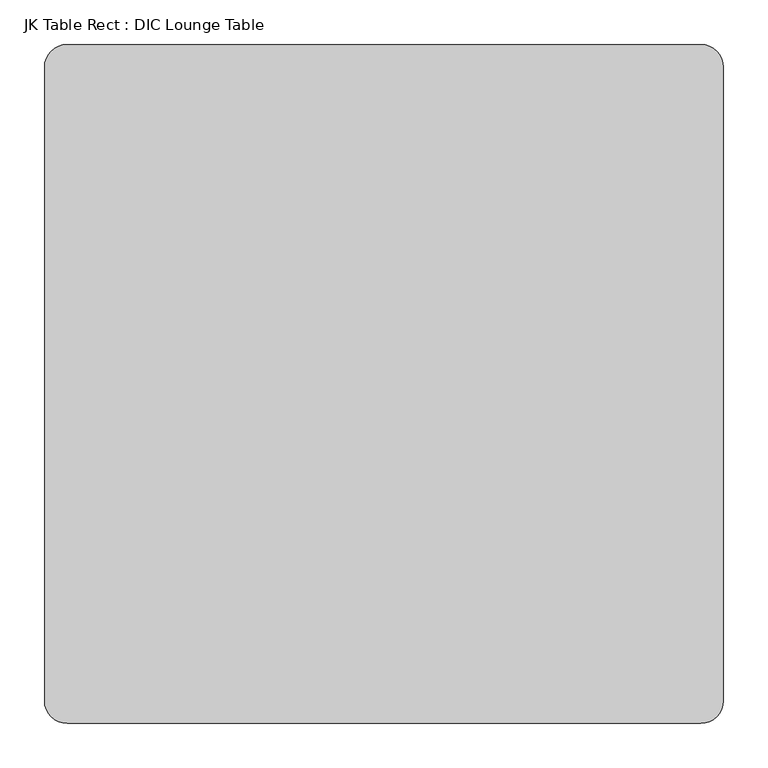
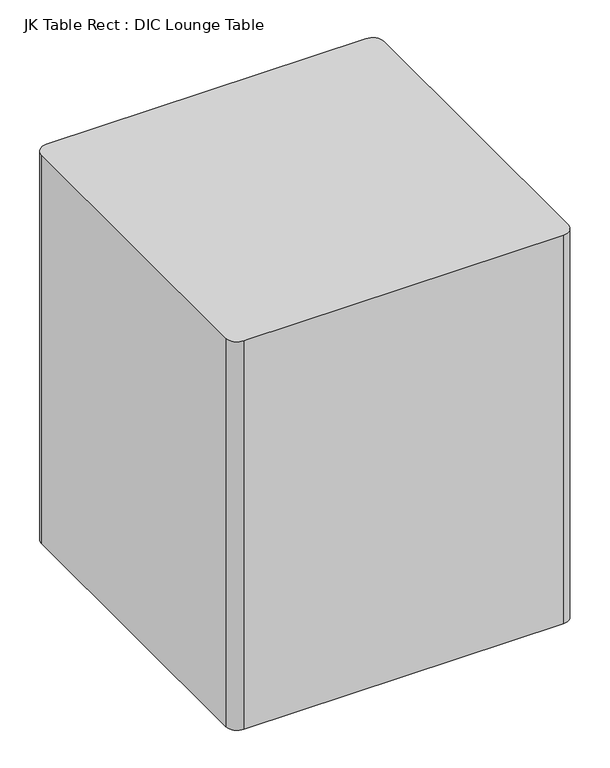
"""IFC4 building model written with IfcOpenShell, lengths in millimetres: furniture geometry, JK Table Rect : DIC Lounge Table."""

import ifcopenshell
import ifcopenshell.guid

model = None  # the IFC model being written
_history = None  # IfcOwnerHistory: only IFC2X3 demands one
_inside = {}  # id of a spatial element -> (the spatial element, [elements in it])
_under = {}  # id of a project, library or spatial element -> (it, [spatial elements below it])
_declared = {}  # id of a project -> (the project, [libraries it declares])
_typed = {}  # id of a type object -> (the type object, [elements of that type])
_made_of = {}  # id of a material, layer set ... -> (it, [elements and type objects made of it])


def new_model(schema):
    """Start an empty IFC model of exactly this schema.

    Asked for "IFC4X3", IfcOpenShell would pick the latest addendum, in which some entities
    have other attributes; the version numbers below select the first issue.
    IFC2X3 requires an IfcOwnerHistory on every rooted entity: one is made here for all.
    """
    global model, _history
    if schema == "IFC4X3":
        model = ifcopenshell.file(schema_version=(4, 3, 0, 0))
    else:
        model = ifcopenshell.file(schema=schema)
    _inside.clear()
    _under.clear()
    _declared.clear()
    _typed.clear()
    _made_of.clear()
    _history = None
    if model.schema == "IFC2X3":
        org = make("IfcOrganization", Name="unknown")
        user = make(
            "IfcPersonAndOrganization",
            ThePerson=make("IfcPerson", FamilyName="unknown"),
            TheOrganization=org,
        )
        app = make(
            "IfcApplication",
            ApplicationDeveloper=org,
            Version="unknown",
            ApplicationFullName="unknown",
            ApplicationIdentifier="unknown",
        )
        _history = make(
            "IfcOwnerHistory",
            OwningUser=user,
            OwningApplication=app,
            ChangeAction="ADDED",
            CreationDate=0,
        )
    return model


def make(cls, **values):
    """One entity of the class cls with the attributes given. An attribute that is None is left unset."""
    return model.create_entity(
        cls, **{name: value for name, value in values.items() if value is not None}
    )


def rooted(cls, **values):
    """An entity with a GlobalId (a new one), such as an element, a storey or a relation."""
    return make(cls, GlobalId=ifcopenshell.guid.new(), OwnerHistory=_history, **values)


def si_unit(unit_type, name, prefix=None):
    """IfcSIUnit, for example si_unit("LENGTHUNIT", "METRE", prefix="MILLI")."""
    return make("IfcSIUnit", UnitType=unit_type, Prefix=prefix, Name=name)


def assignment(units):
    """IfcUnitAssignment: the units of a project."""
    return None if units is None else make("IfcUnitAssignment", Units=units)


def point(xyz):
    """IfcCartesianPoint."""
    return None if xyz is None else make("IfcCartesianPoint", Coordinates=xyz)


def direction(xyz):
    """IfcDirection."""
    return None if xyz is None else make("IfcDirection", DirectionRatios=xyz)


def frame(location, z_axis=None, x_axis=None):
    """IfcAxis2Placement3D, a coordinate frame: its origin and axes. An axis left out is left unset."""
    return make(
        "IfcAxis2Placement3D",
        Location=point(location),
        Axis=direction(z_axis),
        RefDirection=direction(x_axis),
    )


def frame_2d(location, x_axis=None):
    """IfcAxis2Placement2D, a coordinate frame in the plane: its origin and x axis."""
    return make(
        "IfcAxis2Placement2D", Location=point(location), RefDirection=direction(x_axis)
    )


def origin():
    """The frame at (0, 0, 0) with its axes left unset."""
    return frame((0.0, 0.0, 0.0))


def origin_with_axes():
    """The frame at (0, 0, 0) with the z axis (0, 0, 1) and the x axis (1, 0, 0) written out."""
    return frame((0.0, 0.0, 0.0), z_axis=(0.0, 0.0, 1.0), x_axis=(1.0, 0.0, 0.0))


def place(relative_to, where):
    """IfcLocalPlacement: puts the frame where relative to a parent placement (None: the world)."""
    return make(
        "IfcLocalPlacement", PlacementRelTo=relative_to, RelativePlacement=where
    )


def context(
    kind, dimensions, precision=None, world=None, true_north=None, identifier=None
):
    """IfcGeometricRepresentationContext, for example the 3D "Model" context."""
    return make(
        "IfcGeometricRepresentationContext",
        ContextIdentifier=identifier,
        ContextType=kind,
        CoordinateSpaceDimension=dimensions,
        Precision=precision,
        WorldCoordinateSystem=world,
        TrueNorth=true_north,
    )


def project(units=None, contexts=None):
    """IfcProject with its units and contexts."""
    return rooted(
        "IfcProject",
        Name="project",
        RepresentationContexts=contexts,
        UnitsInContext=assignment(units),
    )


def spatial(cls, under=None, at=None, **own):
    """A site, building, storey or space (cls), placed at a placement, below another one or the project."""
    s = rooted(cls, ObjectPlacement=at, **own)
    if under is not None:
        _under.setdefault(under.id(), (under, []))[1].append(s)
    return s


def polyline(points):
    """IfcPolyline through the points."""
    return make("IfcPolyline", Points=[point(p) for p in points])


def circle_curve(where, radius):
    """IfcCircle in the frame where."""
    return make("IfcCircle", Position=where, Radius=radius)


def trimmed(basis, trim1, trim2, sense, master):
    """IfcTrimmedCurve: the piece of a basis curve between two trims."""
    return make(
        "IfcTrimmedCurve",
        BasisCurve=basis,
        Trim1=trim1,
        Trim2=trim2,
        SenseAgreement=sense,
        MasterRepresentation=master,
    )


def segment(curve, same_sense, transition):
    """IfcCompositeCurveSegment."""
    return make(
        "IfcCompositeCurveSegment",
        Transition=transition,
        SameSense=same_sense,
        ParentCurve=curve,
    )


def composite_curve(segments, self_intersect=None):
    """IfcCompositeCurve: segments joined end to end."""
    return make("IfcCompositeCurve", Segments=segments, SelfIntersect=self_intersect)


def outline(outer, holes=None, kind="AREA"):
    """IfcArbitraryClosedProfileDef: a profile drawn as a closed curve; with holes, ...WithVoids."""
    if holes is None:
        return make("IfcArbitraryClosedProfileDef", ProfileType=kind, OuterCurve=outer)
    return make(
        "IfcArbitraryProfileDefWithVoids",
        ProfileType=kind,
        OuterCurve=outer,
        InnerCurves=holes,
    )


def extrude(swept, where, along, depth):
    """IfcExtrudedAreaSolid: the profile swept, set in the frame where, extruded along a direction by depth."""
    return make(
        "IfcExtrudedAreaSolid",
        SweptArea=swept,
        Position=where,
        ExtrudedDirection=direction(along),
        Depth=depth,
    )


def shape(context_of_items, identifier, shape_type, items):
    """IfcShapeRepresentation: the items that make up one representation, for example the "Body"."""
    return make(
        "IfcShapeRepresentation",
        ContextOfItems=context_of_items,
        RepresentationIdentifier=identifier,
        RepresentationType=shape_type,
        Items=items,
    )


def source(mapping_origin, context_of_items, identifier, shape_type, items):
    """IfcRepresentationMap: a shape defined once, which mapped items show again and again."""
    return make(
        "IfcRepresentationMap",
        MappingOrigin=mapping_origin,
        MappedRepresentation=shape(context_of_items, identifier, shape_type, items),
    )


def transform(
    local_origin,
    x_axis=None,
    y_axis=None,
    z_axis=None,
    scale=None,
    scale2=None,
    scale3=None,
    uniform=True,
):
    """IfcCartesianTransformationOperator3D, or its non-uniform kind. x_axis, y_axis, z_axis: its Axis1, 2, 3."""
    if uniform:
        return make(
            "IfcCartesianTransformationOperator3D",
            Axis1=direction(x_axis),
            Axis2=direction(y_axis),
            LocalOrigin=point(local_origin),
            Scale=scale,
            Axis3=direction(z_axis),
        )
    return make(
        "IfcCartesianTransformationOperator3DnonUniform",
        Axis1=direction(x_axis),
        Axis2=direction(y_axis),
        LocalOrigin=point(local_origin),
        Scale=scale,
        Axis3=direction(z_axis),
        Scale2=scale2,
        Scale3=scale3,
    )


def mapped(mapping_source, mapping_target):
    """IfcMappedItem: shows the shape of a source again, moved by a transform."""
    return make(
        "IfcMappedItem", MappingSource=mapping_source, MappingTarget=mapping_target
    )


def made_of(thing, what):
    """Note that an element or type object is made of a material, layer set ...; save() writes the relation."""
    if what is not None:
        _made_of.setdefault(what.id(), (what, []))[1].append(thing)
    return thing


def element(
    cls,
    number,
    at=None,
    inside=None,
    cuts=None,
    type_object=None,
    material=None,
    context=None,
    identifier="Body",
    shape_type=None,
    held_by="IfcProductDefinitionShape",
    body=None,
    shapes=None,
    **own,
):
    """One element of the class cls, such as IfcWall. Its Tag is "e" and its number.

    at: its placement. inside: the storey or other place that contains it. cuts: it is an
    opening in that element (IfcRelVoidsElement). A single representation is given by context,
    identifier, shape_type and body (its items); several are given by shapes. held_by: the class
    of the entity that holds the representations. save() writes the other relations.
    """
    e = rooted(cls, Tag="e%d" % number, ObjectPlacement=at, **own)
    if body is not None:
        shapes = [shape(context, identifier, shape_type, body)]
    if shapes is not None:
        e.Representation = make(held_by, Representations=shapes)
    if inside is not None:
        _inside.setdefault(inside.id(), (inside, []))[1].append(e)
    if cuts is not None:
        rooted(
            "IfcRelVoidsElement", RelatingBuildingElement=cuts, RelatedOpeningElement=e
        )
    if type_object is not None:
        _typed.setdefault(type_object.id(), (type_object, []))[1].append(e)
    return made_of(e, material)


def aggregate(whole, parts):
    """IfcRelAggregates: a whole, such as a stair, and the parts it consists of."""
    return rooted("IfcRelAggregates", RelatingObject=whole, RelatedObjects=parts)


def save(model, path):
    """Write the relations noted so far, then the file.

    IfcRelAggregates (storeys below a building ...), IfcRelContainedInSpatialStructure (elements
    in a storey), IfcRelDefinesByType, IfcRelAssociatesMaterial and IfcRelDeclares: one each for
    every whole, place, type object, material and project.
    """
    for whole, parts in _under.values():
        aggregate(whole, parts)
    for where, things in _inside.values():
        rooted(
            "IfcRelContainedInSpatialStructure",
            RelatedElements=things,
            RelatingStructure=where,
        )
    for kind, things in _typed.values():
        rooted("IfcRelDefinesByType", RelatedObjects=things, RelatingType=kind)
    for what, things in _made_of.values():
        rooted("IfcRelAssociatesMaterial", RelatedObjects=things, RelatingMaterial=what)
    for by, libraries in _declared.values():
        rooted("IfcRelDeclares", RelatingContext=by, RelatedDefinitions=libraries)
    model.write(path)


def jk_table_rect_dic_lounge_table_3608fa95(model_context):
    return source(origin(), model_context, "Body", "SweptSolid", [
        extrude(outline(composite_curve([segment(trimmed(circle_curve(frame_2d((293.6573665, 389.1455296)), 25.4), [point((293.6573665, 414.5455296))], [point((319.0573665, 389.1455296))], False, "CARTESIAN"), True, "CONTINUOUS"), segment(polyline([(319.0573665, 389.1455296), (319.0573665, -322.0544704)]), True, "CONTINUOUS"), segment(trimmed(circle_curve(frame_2d((293.6573665, -322.0544704)), 25.4), [point((319.0573665, -322.0544704))], [point((293.6573665, -347.4544704))], False, "CARTESIAN"), True, "CONTINUOUS"), segment(polyline([(293.6573665, -347.4544704), (-417.5426335, -347.4544704)]), True, "CONTINUOUS"), segment(trimmed(circle_curve(frame_2d((-417.5426335, -322.0544704)), 25.4), [point((-417.5426335, -347.4544704))], [point((-442.9426335, -322.0544704))], False, "CARTESIAN"), True, "CONTINUOUS"), segment(polyline([(-442.9426335, -322.0544704), (-442.9426335, 389.1455296)]), True, "CONTINUOUS"), segment(trimmed(circle_curve(frame_2d((-417.5426335, 389.1455296)), 25.4), [point((-442.9426335, 389.1455296))], [point((-417.5426335, 414.5455296))], False, "CARTESIAN"), True, "CONTINUOUS"), segment(polyline([(-417.5426335, 414.5455296), (293.6573665, 414.5455296)]), True, "CONTINUOUS")], self_intersect=False)), origin_with_axes(), (0.0, 0.0, 1.0), 914.4),
    ])


if __name__ == "__main__":
    model = new_model("IFC4")
    model_context = context("Model", 3, world=origin())
    ifc_project = project(units=[si_unit("LENGTHUNIT", "METRE", prefix="MILLI")], contexts=[model_context])
    site = spatial("IfcSite", under=ifc_project)
    building = spatial("IfcBuilding", under=site)
    placement = place(None, origin())
    jk_table_rect_dic_lounge_table_shape = jk_table_rect_dic_lounge_table_3608fa95(model_context)
    element("IfcFurniture", 1, ObjectType="JK Table Rect : DIC Lounge Table", at=placement, inside=building, context=model_context, shape_type="MappedRepresentation", body=[
        mapped(jk_table_rect_dic_lounge_table_shape, transform((0.0, 0.0, 0.0), x_axis=(1.0, 0.0, 0.0), y_axis=(0.0, 1.0, 0.0), z_axis=(0.0, 0.0, 1.0))),
    ])
    save(model, "model.ifc")

# Revit data of these elements
# Type "JK Table Rect : DIC Lounge Table"
#   Width = 2' - 6"
#   Height = 3' - 0"
#   Depth = 2' - 6"
#   Corner Radius = 0' - 1"
#   Status [instance default] = none
#   Default Elevation = 0
